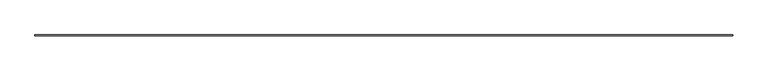
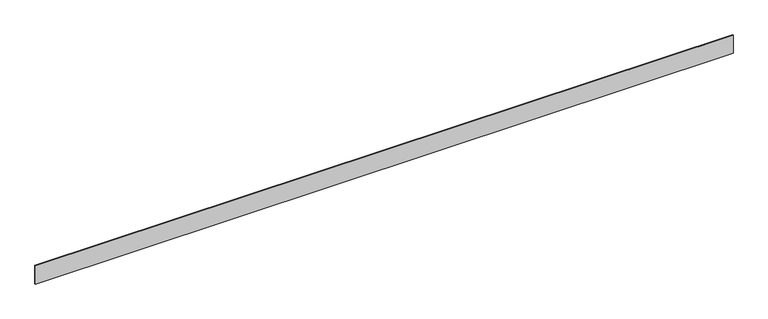
"""IFC4 building model written with IfcOpenShell, lengths in millimetres: proxy geometry, Generic Models 7:Generic Models 1:6:Generic Models 1:6 : Generic Models 7:Generic Models 1:337419:6 : Generic Models 7:Generic Models 1:6:Generic Models 1:6 : Generic Models 7:Generic Models 1:337419:312901."""

from ifc_helpers import new_model, si_unit, frame, origin, place, context, project, spatial, polyline, outline, extrude, source, transform, mapped, element, save


def generic_models_57fde273(model_context):
    return source(origin(), model_context, "Body", "SweptSolid", [
        extrude(outline(polyline([(-536557.2913358, -3.1687897), (-536506.4913358, -5.2854564), (-536506.4913358, -1222.375), (-536557.2913358, -1222.375), (-536557.2913358, -3.1687897)])), frame((557809.7867239, 0.0, 0.0), z_axis=(1.0, 0.0, 0.0), x_axis=(0.0, 1.0, 0.0)), (0.0, 0.0, 1.0), 44500.8),
    ])


if __name__ == "__main__":
    model = new_model("IFC4")
    model_context = context("Model", 3, world=origin())
    ifc_project = project(units=[si_unit("LENGTHUNIT", "METRE", prefix="MILLI")], contexts=[model_context])
    site = spatial("IfcSite", under=ifc_project)
    building = spatial("IfcBuilding", under=site)
    placement = place(None, origin())
    generic_models_shape = generic_models_57fde273(model_context)
    element("IfcBuildingElementProxy", 1, Name="Generic Models 7:Generic Models 1:6:Generic Models 1:6 : Generic Models 7:Generic Models 1:337419:6 : Generic Models 7:Generic Models 1:6:Generic Models 1:6 : Generic Models 7:Generic Models 1:337419:312901", ObjectType="Generic Models 7:Generic Models 1:6:Generic Models 1:6 : Generic Models 7:Generic Models 1:337419:6 : Generic Models 7:Generic Models 1:6:Generic Models 1:6 : Generic Models 7:Generic Models 1:337419:312901", at=placement, inside=building, context=model_context, shape_type="MappedRepresentation", body=[
        mapped(generic_models_shape, transform((0.0, 0.0, 0.0), x_axis=(1.0, 0.0, 0.0), y_axis=(0.0, 1.0, 0.0), z_axis=(0.0, 0.0, 1.0))),
    ])
    save(model, "model.ifc")

# Revit data of these elements
# Type "Generic Models 7:Generic Models 1:6:Generic Models 1:6 : Generic Models 7:Generic Models 1:337419:6 : Generic Models 7:Generic Models 1:6:Generic Models 1:6 : Generic Models 7:Generic Models 1:337419:312901"
#   NameOverride = "Generic Models 7:Generic Models 1:6:Generic Models 1:6 : Generic Models 7:Generic Models 1:337419:312901"
#   ObjectTypeOverride = "Generic Models 1:6 : Generic Models 7:Generic Models 1:337419"
#   Reference = "Generic Models 1"
#   Tag = "312901"
# Element 1 (IfcBuildingElementProxy, "Generic Models 7:Generic Models 1:6:Generic Models 1:6 : Generic Models 7:Generic Models 1:337419:6 : Generic Models 7:Generic Models 1:6:Generic Models 1:6 : Generic Models 7:Generic Models 1:337419:312901")
#   Materials on its faces: "EXTRUDED POLYSTYRENE (XPS) RIGID FOAM INSULATION (FOAMULAR® 250 OR SIMILAR)"
# Materials
#   "EXTRUDED POLYSTYRENE (XPS) RIGID FOAM INSULATION (FOAMULAR® 250 OR SIMILAR)": class "Unassigned", colour RGB 247 185 194, transparency 0, Cost = 0
